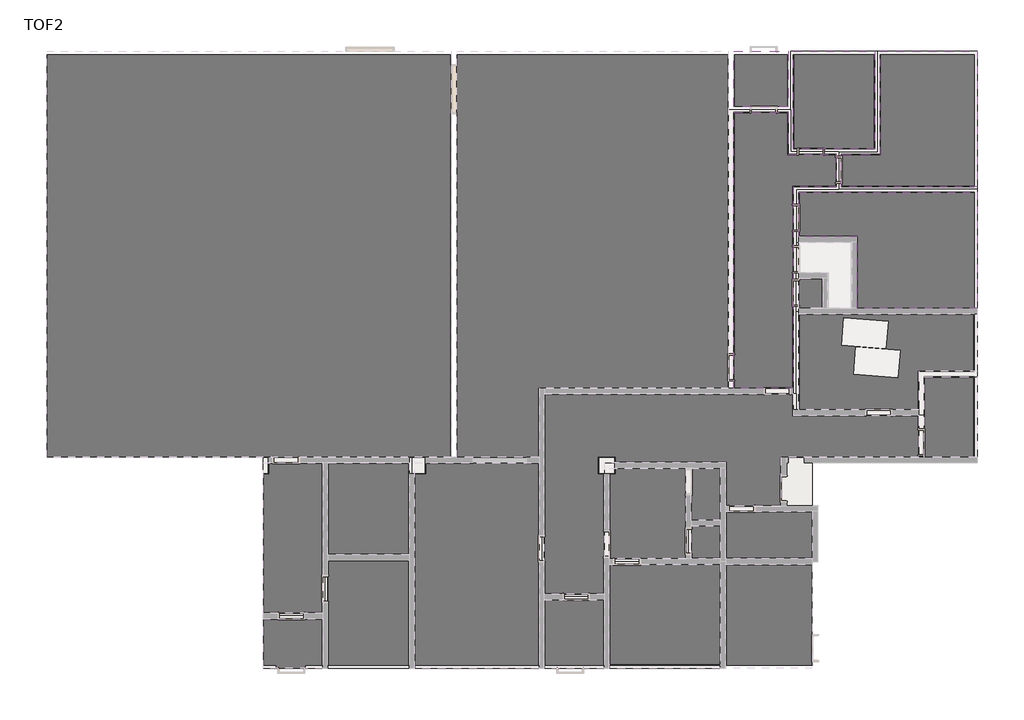
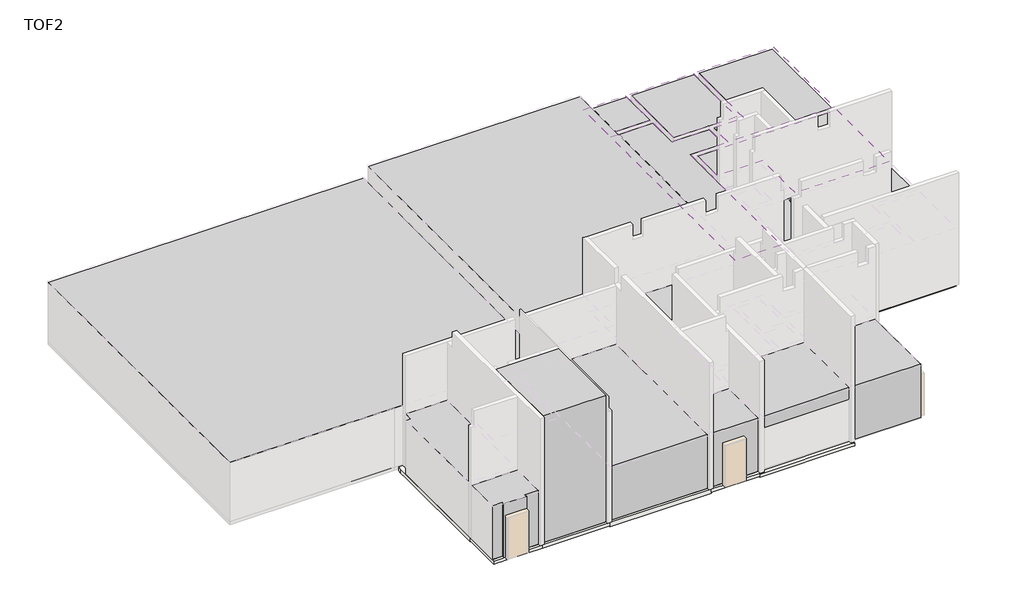
# One storey, part 5 of 5: 24 slabs, 23 proxies, 5 coverings.
"""IFC4 building model written with IfcOpenShell, lengths in millimetres."""

from ifc_helpers import new_model, si_unit, frame, origin, place, context, project, spatial, polyline, outline, extrude, faceted_brep, element, save

model = new_model("IFC4")

# Units and contexts
model_context = context("Model", 3, world=origin())
ifc_project = project(units=[si_unit("LENGTHUNIT", "METRE", prefix="MILLI")], contexts=[model_context])

# Site, building, storey
site = spatial("IfcSite", under=ifc_project)
building = spatial("IfcBuilding", under=site)
storey = spatial("IfcBuildingStorey", under=building, Name="TOF2", Elevation=1149.9618634)

# Proxies
placement = place(None, origin())
element("IfcBuildingElementProxy", 1, Name="Generic Models", at=placement, inside=storey, context=model_context, shape_type="SweptSolid", body=[
    extrude(outline(polyline([(18312.0, 23473.5208589), (33238.0, 23473.5208589), (33238.0, 8611.5208589), (26100.0, 8611.5208589), (18312.0, 8611.5208589), (18312.0, 23473.5208589)])), frame((0.0, 0.0, 1149.9618634), z_axis=(0.0, 0.0, 1.0), x_axis=(1.0, 0.0, 0.0)), (0.0, 0.0, 1.0), 3000.0),
])
element("IfcBuildingElementProxy", 2, Name="Generic Models", at=placement, inside=storey, context=model_context, shape_type="SweptSolid", body=[
    extrude(outline(polyline([(36488.0, 925.5208589), (31912.0, 925.5208589), (31912.0, 4899.0208589), (31912.0, 7987.5208589), (32312.0, 7987.5208589), (32312.0, 8387.5208589), (33350.0, 8387.5208589), (36488.0, 8387.5208589), (36488.0, 3443.8249516), (36488.0, 925.5208589)])), frame((0.0, 0.0, 1156.9618634), z_axis=(0.0, 0.0, 1.0), x_axis=(1.0, 0.0, 0.0)), (0.0, 0.0, 1.0), 2693.0),
])
element("IfcBuildingElementProxy", 3, Name="Generic Models", at=placement, inside=storey, context=model_context, shape_type="SweptSolid", body=[
    extrude(outline(polyline([(33462.0, 23473.5208589), (43488.0, 23473.5208589), (43488.0, 11161.5208589), (36488.0, 11161.5208589), (36488.0, 8611.5208589), (33462.0, 8611.5208589), (33462.0, 23473.5208589)])), frame((0.0, 0.0, 1149.9618634), z_axis=(0.0, 0.0, 1.0), x_axis=(1.0, 0.0, 0.0)), (0.0, 0.0, 1.0), 3500.0),
])
element("IfcBuildingElementProxy", 4, Name="Generic Models", at=placement, inside=storey, context=model_context, shape_type="SweptSolid", body=[
    extrude(outline(polyline([(39107.0, 932.5208589), (39107.0, 3443.8249516), (39107.0, 4642.5208589), (43193.0, 4642.5208589), (43193.0, 932.5208589), (39107.0, 932.5208589)])), frame((0.0, 0.0, 1199.9618634), z_axis=(0.0, 0.0, 1.0), x_axis=(1.0, 0.0, 0.0)), (0.0, 0.0, 1.0), 2650.0),
])
element("IfcBuildingElementProxy", 5, Name="Generic Models", at=placement, inside=storey, context=model_context, shape_type="SweptSolid", body=[
    extrude(outline(polyline([(39307.0, 7992.5208589), (39307.0, 8197.5208589), (41918.0, 8197.5208589), (41918.0, 6174.5208589), (41918.0, 4856.5208589), (39107.0, 4856.5208589), (39107.0, 7992.5208589), (39307.0, 7992.5208589)])), frame((0.0, 0.0, 1149.9618634), z_axis=(0.0, 0.0, 1.0), x_axis=(1.0, 0.0, 0.0)), (0.0, 0.0, 1.0), 2700.0),
])
element("IfcBuildingElementProxy", 6, Name="Generic Models", at=placement, inside=storey, context=model_context, shape_type="SweptSolid", body=[
    extrude(outline(polyline([(42132.0, 8197.5208589), (43193.0, 8197.5208589), (43193.0, 6699.5208589), (43193.0, 6281.5208589), (42132.0, 6281.5208589), (42132.0, 8197.5208589)])), frame((0.0, 0.0, 1199.9618634), z_axis=(0.0, 0.0, 1.0), x_axis=(1.0, 0.0, 0.0)), (0.0, 0.0, 1.0), 2650.0),
])
element("IfcBuildingElementProxy", 7, Name="Generic Models", at=placement, inside=storey, context=model_context, shape_type="SweptSolid", body=[
    extrude(outline(polyline([(43188.0, 4861.5208589), (42137.0, 4861.5208589), (42137.0, 6062.5208589), (43188.0, 6062.5208589), (43188.0, 4861.5208589)])), frame((0.0, 0.0, 1149.9618634), z_axis=(0.0, 0.0, 1.0), x_axis=(1.0, 0.0, 0.0)), (0.0, 0.0, 1.0), 2700.0),
])
element("IfcBuildingElementProxy", 8, Name="Generic Models", at=placement, inside=storey, context=model_context, shape_type="SweptSolid", body=[
    extrude(outline(polyline([(52567.0, 8606.5208589), (50732.0, 8606.5208589), (50732.0, 10249.5208589), (50732.0, 11567.5208589), (52567.0, 11567.5208589), (52567.0, 8606.5208589)])), frame((0.0, 0.0, 1199.9618634), z_axis=(0.0, 0.0, 1.0), x_axis=(1.0, 0.0, 0.0)), (0.0, 0.0, 1.0), 2650.0),
])
element("IfcBuildingElementProxy", 9, Name="Generic Models", at=placement, inside=storey, context=model_context, shape_type="SweptSolid", body=[
    extrude(outline(polyline([(52574.0, 23473.5208589), (52574.0, 18611.5208589), (47687.0, 18611.5208589), (47687.0, 19787.5208589), (49112.0, 19787.5208589), (49112.0, 23473.5208589), (52574.0, 23473.5208589)])), frame((0.0, 0.0, 1156.9618634), z_axis=(0.0, 0.0, 1.0), x_axis=(1.0, 0.0, 0.0)), (0.0, 0.0, 1.0), 2693.0),
])
element("IfcBuildingElementProxy", 10, Name="Generic Models", at=placement, inside=storey, context=model_context, shape_type="SweptSolid", body=[
    extrude(outline(polyline([(43712.0, 23473.5208589), (45688.0, 23473.5208589), (45688.0, 21561.5208589), (43712.0, 21561.5208589), (43712.0, 23473.5208589)])), frame((0.0, 0.0, 1156.9618634), z_axis=(0.0, 0.0, 1.0), x_axis=(1.0, 0.0, 0.0)), (0.0, 0.0, 1.0), 2693.0),
])
element("IfcBuildingElementProxy", 11, Name="Generic Models", at=placement, inside=storey, context=model_context, shape_type="SweptSolid", body=[
    extrude(outline(polyline([(45883.0, 11161.5208589), (43712.0, 11161.5208589), (43712.0, 21337.5208589), (45688.0, 21337.5208589), (45688.0, 19787.5208589), (47463.0, 19787.5208589), (47463.0, 18611.5208589), (45883.0, 18611.5208589), (45883.0, 16649.5208589), (45883.0, 15314.5208589), (45883.0, 13999.5208589), (45883.0, 11161.5208589)])), frame((0.0, 0.0, 1156.9618634), z_axis=(0.0, 0.0, 1.0), x_axis=(1.0, 0.0, 0.0)), (0.0, 0.0, 1.0), 2693.0),
])
element("IfcBuildingElementProxy", 12, Name="Generic Models", at=placement, inside=storey, context=model_context, shape_type="SweptSolid", body=[
    extrude(outline(polyline([(45912.0, 23473.5208589), (48888.0, 23473.5208589), (48888.0, 20011.5208589), (47575.0, 20011.5208589), (45912.0, 20011.5208589), (45912.0, 21449.5208589), (45912.0, 23473.5208589)])), frame((0.0, 0.0, 1156.9618634), z_axis=(0.0, 0.0, 1.0), x_axis=(1.0, 0.0, 0.0)), (0.0, 0.0, 1.0), 2693.0),
])
element("IfcBuildingElementProxy", 13, Name="Generic Models", at=placement, inside=storey, context=model_context, shape_type="SweptSolid", body=[
    extrude(outline(polyline([(50513.0, 10361.5208589), (46107.0, 10361.5208589), (46107.0, 13887.5208589), (52562.0, 13887.5208589), (52562.0, 11786.5208589), (50513.0, 11786.5208589), (50513.0, 10361.5208589)]), holes=[polyline([(47685.4846295, 12746.0331648), (49320.3101517, 12615.8582361), (49401.2726074, 13632.6399633), (47766.4470852, 13762.814892), (47685.4846295, 12746.0331648)]), polyline([(48126.4248192, 11673.6441948), (49761.2503413, 11543.4692661), (49842.212797, 12560.2509933), (48207.3872748, 12690.425922), (48126.4248192, 11673.6441948)])]), frame((0.0, 0.0, 1206.9618634), z_axis=(0.0, 0.0, 1.0), x_axis=(1.0, 0.0, 0.0)), (0.0, 0.0, 1.0), 2643.0),
])
element("IfcBuildingElementProxy", 14, Name="Generic Models", at=placement, inside=storey, context=model_context, shape_type="SweptSolid", body=[
    extrude(outline(polyline([(52574.0, 18387.5208589), (52574.0, 14111.5208589), (48262.0, 14111.5208589), (48262.0, 16761.5208589), (46107.0, 16761.5208589), (46107.0, 18387.5208589), (52574.0, 18387.5208589)])), frame((0.0, 0.0, 1156.9618634), z_axis=(0.0, 0.0, 1.0), x_axis=(1.0, 0.0, 0.0)), (0.0, 0.0, 1.0), 2693.0),
])
element("IfcBuildingElementProxy", 15, Name="Generic Models", at=placement, inside=storey, context=model_context, shape_type="SweptSolid", body=[
    extrude(outline(polyline([(46107.0, 14111.5208589), (46107.0, 15202.5208589), (46963.0, 15202.5208589), (46963.0, 14111.5208589), (46107.0, 14111.5208589)])), frame((0.0, 0.0, 1156.9618634), z_axis=(0.0, 0.0, 1.0), x_axis=(1.0, 0.0, 0.0)), (0.0, 0.0, 1.0), 2693.0),
])
element("IfcBuildingElementProxy", 16, Name="Generic Models", at=placement, inside=storey, context=model_context, shape_type="SweptSolid", body=[
    extrude(outline(polyline([(43412.0, 6587.5208589), (46588.0, 6587.5208589), (46588.0, 4861.5208589), (43412.0, 4861.5208589), (43412.0, 6587.5208589)])), frame((0.0, 0.0, 1156.9618634), z_axis=(0.0, 0.0, 1.0), x_axis=(1.0, 0.0, 0.0)), (0.0, 0.0, 1.0), 2693.0),
])
element("IfcBuildingElementProxy", 17, Name="Generic Models", at=placement, inside=storey, context=model_context, shape_type="SweptSolid", body=[
    extrude(outline(polyline([(46588.0, 925.5208589), (43412.0, 925.5208589), (43412.0, 4637.5208589), (46588.0, 4637.5208589), (46588.0, 925.5208589)])), frame((0.0, 0.0, 1156.9618634), z_axis=(0.0, 0.0, 1.0), x_axis=(1.0, 0.0, 0.0)), (0.0, 0.0, 1.0), 2693.0),
])
element("IfcBuildingElementProxy", 18, Name="Generic Models", at=placement, inside=storey, context=model_context, shape_type="SweptSolid", body=[
    extrude(outline(polyline([(31688.0, 925.5208589), (28712.0, 925.5208589), (28712.0, 4787.0208589), (31688.0, 4787.0208589), (31688.0, 925.5208589)])), frame((0.0, 0.0, 1156.9618634), z_axis=(0.0, 0.0, 1.0), x_axis=(1.0, 0.0, 0.0)), (0.0, 0.0, 1.0), 6343.0),
])
element("IfcBuildingElementProxy", 19, Name="Generic Models", at=placement, inside=storey, context=model_context, shape_type="SweptSolid", body=[
    extrude(outline(polyline([(28712.0, 8387.5208589), (31688.0, 8387.5208589), (31688.0, 7999.5208589), (31688.0, 5011.0208589), (28712.0, 5011.0208589), (28712.0, 8387.5208589)])), frame((0.0, 0.0, 1156.9618634), z_axis=(0.0, 0.0, 1.0), x_axis=(1.0, 0.0, 0.0)), (0.0, 0.0, 1.0), 2693.0),
])
element("IfcBuildingElementProxy", 20, Name="Generic Models", at=placement, inside=storey, context=model_context, shape_type="Brep", body=[
    faceted_brep([(26787.0, 925.5208589, 1156.9618634), (26850.0, 925.5208589, 1156.9618634), (26850.0, 925.5208589, 1149.9618634), (26787.0, 925.5208589, 1149.9618634), (26850.0, 799.5208589, 1156.9618634), (26312.0, 925.5208589, 1156.9618634), (26312.0, 2625.0208589, 1156.9618634), (28488.0, 2625.0208589, 1156.9618634), (28488.0, 925.5208589, 1156.9618634), (27855.0, 925.5208589, 1156.9618634), (27855.0, 799.5208589, 1156.9618634), (26787.0, 925.5208589, 3849.9618634), (26312.0, 925.5208589, 3849.9618634), (26850.0, 799.5208589, 1149.9618634), (26787.0, 799.5208589, 1149.9618634), (26787.0, 799.5208589, 3849.9618634), (27855.0, 799.5208589, 3849.9618634), (26312.0, 2625.0208589, 3849.9618634), (28488.0, 2625.0208589, 3849.9618634), (28488.0, 925.5208589, 3849.9618634), (27855.0, 925.5208589, 3849.9618634)], [[[0, 1, 2, 3]], [[4, 1, 0, 5, 6, 7, 8, 9, 10]], [[11, 12, 5, 0]], [[1, 4, 13, 2]], [[14, 3, 2, 13]], [[3, 14, 15, 11, 0]], [[15, 14, 13, 4, 10, 16]], [[12, 17, 6, 5]], [[17, 18, 7, 6]], [[18, 19, 8, 7]], [[19, 20, 9, 8]], [[20, 16, 10, 9]], [[11, 15, 16, 20, 19, 18, 17, 12]]]),
])
element("IfcBuildingElementProxy", 21, Name="Generic Models", at=placement, inside=storey, context=model_context, shape_type="SweptSolid", body=[
    extrude(outline(polyline([(26512.0, 7987.5208589), (26512.0, 8387.5208589), (28488.0, 8387.5208589), (28488.0, 4899.0208589), (28488.0, 2849.0208589), (26312.0, 2849.0208589), (26312.0, 7987.5208589), (26512.0, 7987.5208589)])), frame((0.0, 0.0, 1156.9618634), z_axis=(0.0, 0.0, 1.0), x_axis=(1.0, 0.0, 0.0)), (0.0, 0.0, 1.0), 2693.0),
])
element("IfcBuildingElementProxy", 22, Name="Generic Models", at=placement, inside=storey, context=model_context, shape_type="SweptSolid", body=[
    extrude(outline(polyline([(39312.0, 8416.5208589), (39312.0, 8611.5208589), (38688.0, 8611.5208589), (38688.0, 7987.5208589), (38888.0, 7987.5208589), (38888.0, 3555.8249516), (36712.0, 3555.8249516), (36712.0, 8499.5208589), (36712.0, 10937.5208589), (43600.0, 10937.5208589), (45883.0, 10937.5208589), (45883.0, 10137.5208589), (50513.0, 10137.5208589), (50513.0, 8611.5208589), (45428.0, 8611.5208589), (45428.0, 6811.5208589), (43412.0, 6811.5208589), (43412.0, 8416.5208589), (39312.0, 8416.5208589)])), frame((0.0, 0.0, 1156.9618634), z_axis=(0.0, 0.0, 1.0), x_axis=(1.0, 0.0, 0.0)), (0.0, 0.0, 1.0), 2693.0),
])
element("IfcBuildingElementProxy", 23, Name="Generic Models", at=placement, inside=storey, context=model_context, shape_type="SweptSolid", body=[
    extrude(outline(polyline([(38888.0, 925.5208589), (36712.0, 925.5208589), (36712.0, 3331.8249516), (38888.0, 3331.8249516), (38888.0, 925.5208589)])), frame((0.0, 0.0, 1156.9618634), z_axis=(0.0, 0.0, 1.0), x_axis=(1.0, 0.0, 0.0)), (0.0, 0.0, 1.0), 2693.0),
])

# Coverings
element("IfcCovering", 24, ObjectType="H_CE_AR_B09_Acoustic Ceiling_T Bar_600x600x9T", at=placement, inside=storey, context=model_context, shape_type="SweptSolid", body=[
    extrude(outline(polyline([(43700.0, 23599.5208589), (45700.0, 23599.5208589), (45700.0, 21549.5208589), (43700.0, 21549.5208589), (43700.0, 23599.5208589)])), frame((0.0, 0.0, 3849.9618634), z_axis=(0.0, 0.0, 1.0), x_axis=(1.0, 0.0, 0.0)), (0.0, 0.0, 1.0), 9.0),
])
element("IfcCovering", 25, ObjectType="H_CE_AR_B09_Acoustic Ceiling_T Bar_600x600x9T", at=placement, inside=storey, context=model_context, shape_type="SweptSolid", body=[
    extrude(outline(polyline([(45900.0, 23599.5208589), (48900.0, 23599.5208589), (48900.0, 19999.5208589), (45900.0, 19999.5208589), (45900.0, 23599.5208589)])), frame((0.0, 0.0, 3849.9618634), z_axis=(0.0, 0.0, 1.0), x_axis=(1.0, 0.0, 0.0)), (0.0, 0.0, 1.0), 9.0),
])
element("IfcCovering", 26, ObjectType="H_CE_AR_B09_Acoustic Ceiling_T Bar_600x600x9T", at=placement, inside=storey, context=model_context, shape_type="SweptSolid", body=[
    extrude(outline(polyline([(49100.0, 23599.5208589), (52700.0, 23599.5208589), (52700.0, 18599.5208589), (47675.0, 18599.5208589), (47675.0, 19799.5208589), (49100.0, 19799.5208589), (49100.0, 23599.5208589)])), frame((0.0, 0.0, 3849.9618634), z_axis=(0.0, 0.0, 1.0), x_axis=(1.0, 0.0, 0.0)), (0.0, 0.0, 1.0), 9.0),
])
element("IfcCovering", 27, ObjectType="H_CE_AR_B09_Acoustic Ceiling_T Bar_600x600x9T", at=placement, inside=storey, context=model_context, shape_type="SweptSolid", body=[
    extrude(outline(polyline([(45895.0, 18599.5208589), (45895.0, 11149.5208589), (43700.0, 11149.5208589), (43700.0, 21349.5208589), (45700.0, 21349.5208589), (45700.0, 19799.5208589), (47475.0, 19799.5208589), (47475.0, 18599.5208589), (45895.0, 18599.5208589)])), frame((0.0, 0.0, 3849.9618634), z_axis=(0.0, 0.0, 1.0), x_axis=(1.0, 0.0, 0.0)), (0.0, 0.0, 1.0), 9.0),
])
element("IfcCovering", 28, ObjectType="H_CE_AR_B09_Acoustic Ceiling_T Bar_600x600x9T", at=placement, inside=storey, context=model_context, shape_type="SweptSolid", body=[
    extrude(outline(polyline([(52700.0, 18399.5208589), (52700.0, 14099.5208589), (48250.0, 14099.5208589), (48250.0, 16749.5208589), (46095.0, 16749.5208589), (46095.0, 18399.5208589), (52700.0, 18399.5208589)])), frame((0.0, 0.0, 3849.9618634), z_axis=(0.0, 0.0, 1.0), x_axis=(1.0, 0.0, 0.0)), (0.0, 0.0, 1.0), 9.0),
])

# Slabs
element("IfcSlab", 29, ObjectType="H_SF_AR_S17_SOG T200_GS1", at=placement, inside=storey, context=model_context, shape_type="Brep", body=[
    faceted_brep([(33350.0, 8599.5208589, 949.9618634), (36600.0, 8599.5208589, 949.9618634), (36600.0, 3443.8249516, 949.9618634), (36600.0, 925.5208589, 949.9618634), (36600.0, 799.5208589, 949.9618634), (31800.0, 799.5208589, 949.9618634), (31800.0, 925.5208589, 949.9618634), (31800.0, 4899.0208589, 949.9618634), (31800.0, 8599.5208589, 949.9618634), (32300.0, 8599.5208589, 949.9618634), (33350.0, 8599.5208589, 1149.9618634), (31800.0, 8599.5208589, 1149.9618634), (31800.0, 4899.0208589, 1149.9618634), (31800.0, 799.5208589, 1149.9618634), (31900.0, 799.5208589, 1149.9618634), (36500.0, 799.5208589, 1149.9618634), (36600.0, 799.5208589, 1149.9618634), (36600.0, 3443.8249516, 1149.9618634), (36600.0, 8599.5208589, 1149.9618634), (36500.0, 8599.5208589, 1149.9618634), (36600.0, 799.5208589, 999.9618634), (31800.0, 799.5208589, 999.9618634)], [[[0, 1, 2, 3, 4, 5, 6, 7, 8, 9]], [[10, 11, 12, 13, 14, 15, 16, 17, 18, 19]], [[1, 0, 10, 19, 18]], [[2, 1, 18, 17]], [[4, 3, 2, 17, 16, 20]], [[5, 4, 20, 16, 15, 14, 13, 21]], [[7, 6, 5, 21, 13, 12]], [[8, 7, 12, 11]], [[0, 9, 8, 11, 10]]]),
])
element("IfcSlab", 30, ObjectType="H_SF_AR_S17_SOG T150_GS1", at=placement, inside=storey, context=model_context, shape_type="Brep", body=[
    faceted_brep([(38900.0, 799.5208589, 949.9618634), (38900.0, 925.5208589, 949.9618634), (38900.0, 3443.8249516, 949.9618634), (38900.0, 4749.5208589, 949.9618634), (42025.0, 4749.5208589, 949.9618634), (43400.0, 4749.5208589, 949.9618634), (43400.0, 4649.5208589, 949.9618634), (43400.0, 925.5208589, 949.9618634), (43400.0, 799.5208589, 949.9618634), (43200.0, 799.5208589, 949.9618634), (38900.0, 799.5208589, 1099.9618634), (43200.0, 799.5208589, 1099.9618634), (43400.0, 799.5208589, 1099.9618634), (43400.0, 925.5208589, 1099.9618634), (43400.0, 4749.5208589, 1099.9618634), (42025.0, 4749.5208589, 1099.9618634), (38900.0, 4749.5208589, 1099.9618634), (38900.0, 3443.8249516, 1099.9618634), (38900.0, 925.5208589, 1099.9618634), (38900.0, 799.5208589, 999.9618634)], [[[0, 1, 2, 3, 4, 5, 6, 7, 8, 9]], [[10, 11, 12, 13, 14, 15, 16, 17, 18]], [[2, 1, 0, 19, 10, 18, 17]], [[3, 2, 17, 16]], [[4, 3, 16, 15]], [[5, 4, 15, 14]], [[8, 7, 6, 5, 14, 13, 12]], [[0, 9, 8, 12, 11, 10, 19]]]),
])
element("IfcSlab", 31, ObjectType="H_SF_AR_S17_SOG T150_GS1", at=placement, inside=storey, context=model_context, shape_type="SweptSolid", body=[
    extrude(outline(polyline([(38900.0, 4749.5208589), (38900.0, 8404.5208589), (42025.0, 8404.5208589), (42025.0, 6174.5208589), (42025.0, 4749.5208589), (38900.0, 4749.5208589)])), frame((0.0, 0.0, 949.9618634), z_axis=(0.0, 0.0, 1.0), x_axis=(1.0, 0.0, 0.0)), (0.0, 0.0, 1.0), 150.0),
])
element("IfcSlab", 32, ObjectType="H_SF_AR_S17_SOG T200_GS1", at=placement, inside=storey, context=model_context, shape_type="Brep", body=[
    faceted_brep([(42025.0, 8404.5208589, 949.9618634), (43400.0, 8404.5208589, 949.9618634), (43400.0, 6699.5208589, 949.9618634), (43400.0, 6174.5208589, 949.9618634), (42025.0, 6174.5208589, 949.9618634), (42025.0, 8404.5208589, 1149.9618634), (42025.0, 6174.5208589, 1149.9618634), (43400.0, 6174.5208589, 1149.9618634), (43400.0, 6699.5208589, 1149.9618634), (43400.0, 8404.5208589, 1149.9618634), (42025.0, 8404.5208589, 1099.9618634), (43400.0, 6174.5208589, 1099.9618634), (42025.0, 6174.5208589, 1099.9618634)], [[[0, 1, 2, 3, 4]], [[5, 6, 7, 8, 9]], [[1, 0, 10, 5, 9]], [[2, 1, 9, 8]], [[3, 2, 8, 7, 11]], [[4, 3, 11, 7, 6, 12]], [[0, 4, 12, 6, 5, 10]]]),
])
element("IfcSlab", 33, ObjectType="H_SF_AR_S17_SOG T150_GS1", at=placement, inside=storey, context=model_context, shape_type="Brep", body=[
    faceted_brep([(43400.0, 4749.5208589, 949.9618634), (42025.0, 4749.5208589, 949.9618634), (42025.0, 6174.5208589, 949.9618634), (43400.0, 6174.5208589, 949.9618634), (43400.0, 4849.5208589, 949.9618634), (43400.0, 4749.5208589, 1099.9618634), (43400.0, 4849.5208589, 1099.9618634), (43400.0, 6174.5208589, 1099.9618634), (42025.0, 6174.5208589, 1099.9618634), (42025.0, 4749.5208589, 1099.9618634)], [[[0, 1, 2, 3, 4]], [[5, 6, 7, 8, 9]], [[1, 0, 5, 9]], [[2, 1, 9, 8]], [[3, 2, 8, 7]], [[0, 4, 3, 7, 6, 5]]]),
])
element("IfcSlab", 34, ObjectType="H_SF_AR_S17_SOG T150_GS1", at=placement, inside=storey, context=model_context, shape_type="Brep", body=[
    faceted_brep([(52700.0, 8599.5208589, 949.9618634), (52574.0, 8599.5208589, 949.9618634), (50725.0, 8599.5208589, 949.9618634), (50725.0, 10149.5208589, 949.9618634), (50725.0, 10249.5208589, 949.9618634), (50725.0, 11574.5208589, 949.9618634), (52574.0, 11574.5208589, 949.9618634), (52700.0, 11574.5208589, 949.9618634), (52700.0, 8599.5208589, 1099.9618634), (52700.0, 11574.5208589, 1099.9618634), (52574.0, 11574.5208589, 1099.9618634), (50725.0, 11574.5208589, 1099.9618634), (50725.0, 10249.5208589, 1099.9618634), (50725.0, 8599.5208589, 1099.9618634), (52574.0, 8599.5208589, 1099.9618634), (50725.0, 11574.5208589, 999.9618634), (52700.0, 11574.5208589, 999.9618634)], [[[0, 1, 2, 3, 4, 5, 6, 7]], [[8, 9, 10, 11, 12, 13, 14]], [[2, 1, 0, 8, 14, 13]], [[4, 3, 2, 13, 12]], [[5, 4, 12, 11, 15]], [[7, 6, 5, 15, 11, 10, 9, 16]], [[0, 7, 16, 9, 8]]]),
])
element("IfcSlab", 35, ObjectType="H_SF_AR_S17_SOG T150_GS1", at=placement, inside=storey, context=model_context, shape_type="Brep", body=[
    faceted_brep([(52700.0, 18499.5208589, 999.9618634), (47575.0, 18499.5208589, 999.9618634), (47575.0, 19899.5208589, 999.9618634), (49000.0, 19899.5208589, 999.9618634), (49000.0, 23599.5208589, 999.9618634), (49100.0, 23599.5208589, 999.9618634), (52574.0, 23599.5208589, 999.9618634), (52700.0, 23599.5208589, 999.9618634), (52700.0, 18599.5208589, 999.9618634), (52700.0, 18499.5208589, 1149.9618634), (52700.0, 18599.5208589, 1149.9618634), (52700.0, 23599.5208589, 1149.9618634), (52574.0, 23599.5208589, 1149.9618634), (49100.0, 23599.5208589, 1149.9618634), (49000.0, 23599.5208589, 1149.9618634), (49000.0, 19899.5208589, 1149.9618634), (47575.0, 19899.5208589, 1149.9618634), (47575.0, 18499.5208589, 1149.9618634)], [[[0, 1, 2, 3, 4, 5, 6, 7, 8]], [[9, 10, 11, 12, 13, 14, 15, 16, 17]], [[1, 0, 9, 17]], [[2, 1, 17, 16]], [[3, 2, 16, 15]], [[4, 3, 15, 14]], [[7, 6, 5, 4, 14, 13, 12, 11]], [[0, 8, 7, 11, 10, 9]]]),
])
element("IfcSlab", 36, ObjectType="H_SF_AR_S17_SOG T150_GS1", at=placement, inside=storey, context=model_context, shape_type="Brep", body=[
    faceted_brep([(46000.0, 10949.5208589, 999.9618634), (43500.0, 10949.5208589, 999.9618634), (43500.0, 11149.5208589, 999.9618634), (43500.0, 21449.5208589, 999.9618634), (43700.0, 21449.5208589, 999.9618634), (45800.0, 21449.5208589, 999.9618634), (45800.0, 19899.5208589, 999.9618634), (47575.0, 19899.5208589, 999.9618634), (47575.0, 18499.5208589, 999.9618634), (46000.0, 18499.5208589, 999.9618634), (46000.0, 16649.5208589, 999.9618634), (46000.0, 16549.5208589, 999.9618634), (46000.0, 15414.5208589, 999.9618634), (46000.0, 15412.0208589, 999.9618634), (46000.0, 15314.5208589, 999.9618634), (46000.0, 13999.5208589, 999.9618634), (46000.0, 11149.5208589, 999.9618634), (46000.0, 10949.5208589, 1149.9618634), (46000.0, 13999.5208589, 1149.9618634), (46000.0, 15314.5208589, 1149.9618634), (46000.0, 15412.0208589, 1149.9618634), (46000.0, 16412.0208589, 1149.9618634), (46000.0, 16549.5208589, 1149.9618634), (46000.0, 16649.5208589, 1149.9618634), (46000.0, 18499.5208589, 1149.9618634), (47575.0, 18499.5208589, 1149.9618634), (47575.0, 19899.5208589, 1149.9618634), (45800.0, 19899.5208589, 1149.9618634), (45800.0, 21449.5208589, 1149.9618634), (43700.0, 21449.5208589, 1149.9618634), (43500.0, 21449.5208589, 1149.9618634), (43500.0, 12424.5208589, 1149.9618634), (43500.0, 11424.5208589, 1149.9618634), (43500.0, 11149.5208589, 1149.9618634), (43500.0, 10949.5208589, 1149.9618634), (44800.0, 10949.5208589, 1149.9618634), (45800.0, 10949.5208589, 1149.9618634), (45895.0, 10949.5208589, 1149.9618634)], [[[0, 1, 2, 3, 4, 5, 6, 7, 8, 9, 10, 11, 12, 13, 14, 15, 16]], [[17, 18, 19, 20, 21, 22, 23, 24, 25, 26, 27, 28, 29, 30, 31, 32, 33, 34, 35, 36, 37]], [[1, 0, 17, 37, 36, 35, 34]], [[3, 2, 1, 34, 33, 32, 31, 30]], [[5, 4, 3, 30, 29, 28]], [[6, 5, 28, 27]], [[7, 6, 27, 26]], [[8, 7, 26, 25]], [[9, 8, 25, 24]], [[10, 9, 24, 23]], [[14, 13, 12, 11, 10, 23, 22, 21, 20, 19]], [[15, 14, 19, 18]], [[0, 16, 15, 18, 17]]]),
])
element("IfcSlab", 37, ObjectType="H_SF_AR_S17_SOG T150_GS1", at=placement, inside=storey, context=model_context, shape_type="Brep", body=[
    faceted_brep([(47575.0, 19899.5208589, 999.9618634), (45800.0, 19899.5208589, 999.9618634), (45800.0, 21449.5208589, 999.9618634), (45800.0, 23599.5208589, 999.9618634), (45900.0, 23599.5208589, 999.9618634), (48900.0, 23599.5208589, 999.9618634), (49000.0, 23599.5208589, 999.9618634), (49000.0, 19899.5208589, 999.9618634), (45800.0, 19899.5208589, 1149.9618634), (47575.0, 19899.5208589, 1149.9618634), (49000.0, 19899.5208589, 1149.9618634), (49000.0, 23599.5208589, 1149.9618634), (48900.0, 23599.5208589, 1149.9618634), (45900.0, 23599.5208589, 1149.9618634), (45800.0, 23599.5208589, 1149.9618634), (45800.0, 21449.5208589, 1149.9618634)], [[[0, 1, 2, 3, 4, 5, 6, 7]], [[8, 9, 10, 11, 12, 13, 14, 15]], [[1, 0, 9, 8]], [[2, 1, 8, 15]], [[3, 2, 15, 14]], [[6, 5, 4, 3, 14, 13, 12, 11]], [[7, 6, 11, 10]], [[0, 7, 10, 9]]]),
])
element("IfcSlab", 38, ObjectType="H_SF_AR_S17_SOG T150_GS1", at=placement, inside=storey, context=model_context, shape_type="Brep", body=[
    faceted_brep([(50725.0, 10149.5208589, 999.9618634), (50525.0, 10149.5208589, 999.9618634), (46000.0, 10149.5208589, 999.9618634), (46000.0, 10349.5208589, 999.9618634), (46000.0, 10949.5208589, 999.9618634), (46000.0, 11049.5208589, 999.9618634), (46000.0, 11149.5208589, 999.9618634), (46000.0, 13999.5208589, 999.9618634), (47075.0, 13999.5208589, 999.9618634), (47175.0, 13999.5208589, 999.9618634), (48050.0, 13999.5208589, 999.9618634), (48150.0, 13999.5208589, 999.9618634), (52700.0, 13999.5208589, 999.9618634), (52700.0, 11774.5208589, 999.9618634), (52700.0, 11574.5208589, 999.9618634), (50725.0, 11574.5208589, 999.9618634), (50725.0, 10249.5208589, 999.9618634), (46000.0, 10149.5208589, 1149.9618634), (50725.0, 10149.5208589, 1149.9618634), (50725.0, 11574.5208589, 1149.9618634), (52700.0, 11574.5208589, 1149.9618634), (52700.0, 11774.5208589, 1149.9618634), (52700.0, 13899.5208589, 1149.9618634), (52700.0, 13999.5208589, 1149.9618634), (48150.0, 13999.5208589, 1149.9618634), (48050.0, 13999.5208589, 1149.9618634), (47175.0, 13999.5208589, 1149.9618634), (47075.0, 13999.5208589, 1149.9618634), (46000.0, 13999.5208589, 1149.9618634), (46000.0, 11049.5208589, 1149.9618634), (46000.0, 10949.5208589, 1149.9618634), (50725.0, 10149.5208589, 1099.9618634), (52700.0, 11574.5208589, 1099.9618634), (50725.0, 11574.5208589, 1099.9618634)], [[[0, 1, 2, 3, 4, 5, 6, 7, 8, 9, 10, 11, 12, 13, 14, 15, 16]], [[17, 18, 19, 20, 21, 22, 23, 24, 25, 26, 27, 28, 29, 30]], [[2, 1, 0, 31, 18, 17]], [[2, 17, 30, 29, 5, 4, 3]], [[7, 6, 5, 29, 28]], [[8, 7, 28, 27]], [[11, 10, 9, 8, 27, 26, 25, 24]], [[12, 11, 24, 23]], [[14, 13, 12, 23, 22, 21, 20, 32]], [[15, 14, 32, 20, 19, 33]], [[19, 18, 31, 0, 16, 15, 33]]]),
])
element("IfcSlab", 39, ObjectType="H_SF_AR_S17_SOG T150_GS1", at=placement, inside=storey, context=model_context, shape_type="Brep", body=[
    faceted_brep([(46000.0, 18499.5208589, 999.9618634), (47575.0, 18499.5208589, 999.9618634), (52700.0, 18499.5208589, 999.9618634), (52700.0, 18399.5208589, 999.9618634), (52700.0, 13999.5208589, 999.9618634), (48050.0, 13999.5208589, 999.9618634), (48050.0, 16549.5208589, 999.9618634), (46095.0, 16549.5208589, 999.9618634), (46000.0, 16549.5208589, 999.9618634), (46000.0, 16649.5208589, 999.9618634), (47575.0, 18499.5208589, 1149.9618634), (46000.0, 18499.5208589, 1149.9618634), (46000.0, 16649.5208589, 1149.9618634), (46000.0, 16549.5208589, 1149.9618634), (46095.0, 16549.5208589, 1149.9618634), (48050.0, 16549.5208589, 1149.9618634), (48050.0, 13999.5208589, 1149.9618634), (52700.0, 13999.5208589, 1149.9618634), (52700.0, 14099.5208589, 1149.9618634), (52700.0, 18399.5208589, 1149.9618634), (52700.0, 18499.5208589, 1149.9618634), (46000.0, 16549.5208589, 1099.9618634), (48050.0, 13999.5208589, 1099.9618634), (48050.0, 16549.5208589, 1099.9618634)], [[[0, 1, 2, 3, 4, 5, 6, 7, 8, 9]], [[10, 11, 12, 13, 14, 15, 16, 17, 18, 19, 20]], [[11, 0, 9, 8, 21, 13, 12]], [[1, 0, 11, 10]], [[2, 1, 10, 20]], [[4, 3, 2, 20, 19, 18, 17]], [[5, 4, 17, 16, 22]], [[6, 5, 22, 16, 15, 23]], [[8, 7, 6, 23, 15, 14, 13, 21]]]),
])
element("IfcSlab", 40, ObjectType="H_SF_AR_S17_SOG T150_GS1", at=placement, inside=storey, context=model_context, shape_type="Brep", body=[
    faceted_brep([(46000.0, 15414.5208589, 949.9618634), (46000.0, 16549.5208589, 949.9618634), (46095.0, 16549.5208589, 949.9618634), (48050.0, 16549.5208589, 949.9618634), (48050.0, 13999.5208589, 949.9618634), (47175.0, 13999.5208589, 949.9618634), (47175.0, 15414.5208589, 949.9618634), (46095.0, 15414.5208589, 949.9618634), (46000.0, 16549.5208589, 1099.9618634), (46000.0, 15414.5208589, 1099.9618634), (46095.0, 15414.5208589, 1099.9618634), (47175.0, 15414.5208589, 1099.9618634), (47175.0, 13999.5208589, 1099.9618634), (48050.0, 13999.5208589, 1099.9618634), (48050.0, 16549.5208589, 1099.9618634), (46095.0, 16549.5208589, 1099.9618634), (46000.0, 15414.5208589, 999.9618634), (46000.0, 16549.5208589, 999.9618634), (48050.0, 16549.5208589, 999.9618634), (48050.0, 13999.5208589, 999.9618634), (47175.0, 13999.5208589, 999.9618634)], [[[0, 1, 2, 3, 4, 5, 6, 7]], [[8, 9, 10, 11, 12, 13, 14, 15]], [[1, 0, 16, 9, 8, 17]], [[3, 2, 1, 17, 8, 15, 14, 18]], [[4, 3, 18, 14, 13, 19]], [[5, 4, 19, 13, 12, 20]], [[6, 5, 20, 12, 11]], [[0, 7, 6, 11, 10, 9, 16]]]),
])
element("IfcSlab", 41, ObjectType="H_SF_AR_S17_SOG T150_GS1", at=placement, inside=storey, context=model_context, shape_type="Brep", body=[
    faceted_brep([(46000.0, 15412.0208589, 999.9618634), (46095.0, 15412.0208589, 999.9618634), (47175.0, 15412.0208589, 999.9618634), (47175.0, 13999.5208589, 999.9618634), (46000.0, 13999.5208589, 999.9618634), (46000.0, 15314.5208589, 999.9618634), (47175.0, 15412.0208589, 1149.9618634), (46095.0, 15412.0208589, 1149.9618634), (46000.0, 15412.0208589, 1149.9618634), (46000.0, 15314.5208589, 1149.9618634), (46000.0, 13999.5208589, 1149.9618634), (47175.0, 13999.5208589, 1149.9618634), (47175.0, 15214.5208589, 1149.9618634), (47175.0, 15412.0208589, 1099.9618634), (47175.0, 13999.5208589, 1099.9618634)], [[[0, 1, 2, 3, 4, 5]], [[6, 7, 8, 9, 10, 11, 12]], [[8, 0, 5, 4, 10, 9]], [[2, 1, 0, 8, 7, 6, 13]], [[3, 2, 13, 6, 12, 11, 14]], [[4, 3, 14, 11, 10]]]),
])
element("IfcSlab", 42, ObjectType="H_SF_AR_S17_SOG T150_GS1", at=placement, inside=storey, context=model_context, shape_type="Brep", body=[
    faceted_brep([(31800.0, 4899.0208589, 999.9618634), (31800.0, 925.5208589, 999.9618634), (31800.0, 799.5208589, 999.9618634), (28600.0, 799.5208589, 999.9618634), (28600.0, 2737.0208589, 999.9618634), (28600.0, 4899.0208589, 999.9618634), (31800.0, 4899.0208589, 1149.9618634), (28600.0, 4899.0208589, 1149.9618634), (28600.0, 2737.0208589, 1149.9618634), (28600.0, 799.5208589, 1149.9618634), (28700.0, 799.5208589, 1149.9618634), (31700.0, 799.5208589, 1149.9618634), (31800.0, 799.5208589, 1149.9618634)], [[[0, 1, 2, 3, 4, 5]], [[6, 7, 8, 9, 10, 11, 12]], [[2, 1, 0, 6, 12]], [[3, 2, 12, 11, 10, 9]], [[4, 3, 9, 8]], [[5, 4, 8, 7]], [[0, 5, 7, 6]]]),
])
element("IfcSlab", 43, ObjectType="H_SF_AR_S17_SOG T200_GS1", at=placement, inside=storey, context=model_context, shape_type="Brep", body=[
    faceted_brep([(28600.0, 8599.5208589, 949.9618634), (31700.0, 8599.5208589, 949.9618634), (31800.0, 8599.5208589, 949.9618634), (31800.0, 4899.0208589, 949.9618634), (28600.0, 4899.0208589, 949.9618634), (28600.0, 8599.5208589, 1149.9618634), (28600.0, 4899.0208589, 1149.9618634), (31800.0, 4899.0208589, 1149.9618634), (31800.0, 8599.5208589, 1149.9618634), (31800.0, 4899.0208589, 999.9618634), (28600.0, 4899.0208589, 999.9618634)], [[[0, 1, 2, 3, 4]], [[5, 6, 7, 8]], [[2, 1, 0, 5, 8]], [[3, 2, 8, 7, 9]], [[4, 3, 9, 7, 6, 10]], [[0, 4, 10, 6, 5]]]),
])
element("IfcSlab", 44, ObjectType="H_SF_AR_S17_SOG T150_GS1", at=placement, inside=storey, context=model_context, shape_type="Brep", body=[
    faceted_brep([(26300.0, 799.5208589, 999.9618634), (26300.0, 925.5208589, 999.9618634), (26300.0, 2737.0208589, 999.9618634), (26500.0, 2737.0208589, 999.9618634), (28600.0, 2737.0208589, 999.9618634), (28600.0, 799.5208589, 999.9618634), (27855.0, 799.5208589, 999.9618634), (26850.0, 799.5208589, 999.9618634), (26724.0, 799.5208589, 999.9618634), (26500.0, 799.5208589, 999.9618634), (26300.0, 799.5208589, 1149.9618634), (26724.0, 799.5208589, 1149.9618634), (26850.0, 799.5208589, 1149.9618634), (27850.0, 799.5208589, 1149.9618634), (27855.0, 799.5208589, 1149.9618634), (28500.0, 799.5208589, 1149.9618634), (28600.0, 799.5208589, 1149.9618634), (28600.0, 2737.0208589, 1149.9618634), (26300.0, 2737.0208589, 1149.9618634), (26300.0, 925.5208589, 1149.9618634)], [[[0, 1, 2, 3, 4, 5, 6, 7, 8, 9]], [[10, 11, 12, 13, 14, 15, 16, 17, 18, 19]], [[2, 1, 0, 10, 19, 18]], [[4, 3, 2, 18, 17]], [[5, 4, 17, 16]], [[0, 9, 8, 7, 6, 5, 16, 15, 14, 13, 12, 11, 10]]]),
])
element("IfcSlab", 45, ObjectType="H_SF_AR_S17_SOG T200_GS1", at=placement, inside=storey, context=model_context, shape_type="Brep", body=[
    faceted_brep([(26300.0, 8599.5208589, 949.9618634), (26500.0, 8599.5208589, 949.9618634), (28600.0, 8599.5208589, 949.9618634), (28600.0, 4899.0208589, 949.9618634), (28600.0, 2737.0208589, 949.9618634), (26500.0, 2737.0208589, 949.9618634), (26300.0, 2737.0208589, 949.9618634), (26300.0, 7999.5208589, 949.9618634), (26300.0, 8397.9255867, 949.9618634), (26300.0, 8599.5208589, 1149.9618634), (26300.0, 8397.9255867, 1149.9618634), (26300.0, 2737.0208589, 1149.9618634), (28600.0, 2737.0208589, 1149.9618634), (28600.0, 4899.0208589, 1149.9618634), (28600.0, 8599.5208589, 1149.9618634), (27650.0, 8599.5208589, 1149.9618634), (26650.0, 8599.5208589, 1149.9618634), (28600.0, 2737.0208589, 999.9618634), (26300.0, 2737.0208589, 999.9618634)], [[[0, 1, 2, 3, 4, 5, 6, 7, 8]], [[9, 10, 11, 12, 13, 14, 15, 16]], [[2, 1, 0, 9, 16, 15, 14]], [[3, 2, 14, 13]], [[4, 3, 13, 12, 17]], [[6, 5, 4, 17, 12, 11, 18]], [[8, 7, 6, 18, 11, 10]], [[0, 8, 10, 9]]]),
])
element("IfcSlab", 46, ObjectType="H_SF_AR_S17_SOG T200_GS1", at=placement, inside=storey, context=model_context, shape_type="Brep", body=[
    faceted_brep([(36600.0, 8499.5208589, 949.9618634), (36600.0, 8599.5208589, 949.9618634), (36600.0, 10799.5208589, 949.9618634), (36600.0, 11149.5208589, 949.9618634), (43500.0, 11149.5208589, 949.9618634), (43600.0, 11149.5208589, 949.9618634), (43700.0, 11149.5208589, 949.9618634), (45895.0, 11149.5208589, 949.9618634), (46000.0, 11149.5208589, 949.9618634), (46000.0, 10349.5208589, 949.9618634), (46000.0, 10149.5208589, 949.9618634), (50525.0, 10149.5208589, 949.9618634), (50725.0, 10149.5208589, 949.9618634), (50725.0, 8599.5208589, 949.9618634), (50525.0, 8599.5208589, 949.9618634), (46600.0, 8599.5208589, 949.9618634), (46600.0, 8399.5208589, 949.9618634), (46600.0, 8387.5208589, 949.9618634), (46600.0, 4849.5208589, 949.9618634), (46600.0, 4649.5208589, 949.9618634), (43400.0, 4649.5208589, 949.9618634), (43400.0, 4749.5208589, 949.9618634), (43400.0, 4849.5208589, 949.9618634), (43400.0, 6174.5208589, 949.9618634), (43400.0, 6699.5208589, 949.9618634), (43400.0, 8404.5208589, 949.9618634), (42025.0, 8404.5208589, 949.9618634), (38900.0, 8404.5208589, 949.9618634), (38900.0, 4749.5208589, 949.9618634), (38900.0, 3443.8249516, 949.9618634), (36600.0, 3443.8249516, 949.9618634), (36600.0, 11149.5208589, 1149.9618634), (36600.0, 10799.5208589, 1149.9618634), (36600.0, 8599.5208589, 1149.9618634), (36600.0, 8499.5208589, 1149.9618634), (36600.0, 3443.8249516, 1149.9618634), (38900.0, 3443.8249516, 1149.9618634), (38900.0, 4749.5208589, 1149.9618634), (38900.0, 8404.5208589, 1149.9618634), (42025.0, 8404.5208589, 1149.9618634), (43400.0, 8404.5208589, 1149.9618634), (43400.0, 6699.5208589, 1149.9618634), (43400.0, 6174.5208589, 1149.9618634), (43400.0, 4849.5208589, 1149.9618634), (43400.0, 4649.5208589, 1149.9618634), (46600.0, 4649.5208589, 1149.9618634), (46600.0, 4749.5208589, 1149.9618634), (46600.0, 4849.5208589, 1149.9618634), (46600.0, 8387.5208589, 1149.9618634), (46600.0, 8399.5208589, 1149.9618634), (46600.0, 8599.5208589, 1149.9618634), (50525.0, 8599.5208589, 1149.9618634), (50725.0, 8599.5208589, 1149.9618634), (50725.0, 8649.5208589, 1149.9618634), (50725.0, 9649.5208589, 1149.9618634), (50725.0, 10149.5208589, 1149.9618634), (46000.0, 10149.5208589, 1149.9618634), (46000.0, 10949.5208589, 1149.9618634), (43500.0, 10949.5208589, 1149.9618634), (43500.0, 11149.5208589, 1149.9618634), (36700.0, 11149.5208589, 1149.9618634), (43500.0, 11149.5208589, 1049.9618634), (43500.0, 11149.5208589, 999.9618634), (43600.0, 11149.5208589, 999.9618634), (43700.0, 11149.5208589, 999.9618634), (45895.0, 11149.5208589, 999.9618634), (46000.0, 11149.5208589, 999.9618634), (46000.0, 10949.5208589, 999.9618634), (46000.0, 10149.5208589, 999.9618634), (50725.0, 10149.5208589, 999.9618634), (50725.0, 8599.5208589, 1099.9618634), (43400.0, 4649.5208589, 1099.9618634), (42025.0, 8404.5208589, 1099.9618634), (38900.0, 8404.5208589, 1099.9618634), (38900.0, 4749.5208589, 1099.9618634), (38900.0, 3443.8249516, 1099.9618634), (38900.0, 3443.8249516, 999.9618634), (36600.0, 3443.8249516, 999.9618634), (43500.0, 10949.5208589, 999.9618634)], [[[0, 1, 2, 3, 4, 5, 6, 7, 8, 9, 10, 11, 12, 13, 14, 15, 16, 17, 18, 19, 20, 21, 22, 23, 24, 25, 26, 27, 28, 29, 30]], [[31, 32, 33, 34, 35, 36, 37, 38, 39, 40, 41, 42, 43, 44, 45, 46, 47, 48, 49, 50, 51, 52, 53, 54, 55, 56, 57, 58, 59, 60]], [[3, 2, 1, 0, 34, 33, 32, 31]], [[5, 4, 3, 31, 60, 59, 61, 62, 63]], [[8, 7, 6, 5, 63, 64, 65, 66]], [[10, 9, 8, 66, 67, 57, 56, 68]], [[12, 11, 10, 68, 56, 55, 69]], [[13, 12, 69, 55, 54, 53, 52, 70]], [[15, 14, 13, 70, 52, 51, 50]], [[19, 18, 17, 16, 15, 50, 49, 48, 47, 46, 45]], [[20, 19, 45, 44, 71]], [[40, 25, 24, 23, 22, 21, 20, 71, 44, 43, 42, 41]], [[26, 25, 40, 39, 72]], [[27, 26, 72, 39, 38, 73]], [[28, 27, 73, 38, 37, 74]], [[29, 28, 74, 37, 36, 75, 76]], [[30, 29, 76, 75, 36, 35, 77]], [[0, 30, 77, 35, 34]], [[78, 67, 66, 65, 64, 63, 62]], [[67, 78, 58, 57]], [[58, 78, 62, 61, 59]]]),
])
element("IfcSlab", 47, ObjectType="H_SF_AR_S17_SOG T150_GS1", at=placement, inside=storey, context=model_context, shape_type="Brep", body=[
    faceted_brep([(36600.0, 799.5208589, 999.9618634), (36600.0, 925.5208589, 999.9618634), (36600.0, 3443.8249516, 999.9618634), (38900.0, 3443.8249516, 999.9618634), (38900.0, 925.5208589, 999.9618634), (38900.0, 799.5208589, 999.9618634), (36600.0, 799.5208589, 1149.9618634), (36700.0, 799.5208589, 1149.9618634), (37155.0, 799.5208589, 1149.9618634), (38155.0, 799.5208589, 1149.9618634), (38900.0, 799.5208589, 1149.9618634), (38900.0, 925.5208589, 1149.9618634), (38900.0, 3443.8249516, 1149.9618634), (36600.0, 3443.8249516, 1149.9618634), (38900.0, 799.5208589, 1099.9618634)], [[[0, 1, 2, 3, 4, 5]], [[6, 7, 8, 9, 10, 11, 12, 13]], [[2, 1, 0, 6, 13]], [[3, 2, 13, 12]], [[5, 4, 3, 12, 11, 10, 14]], [[0, 5, 14, 10, 9, 8, 7, 6]]]),
])
element("IfcSlab", 48, ObjectType="H_FL_AR_B07_Vinyl Tile", at=placement, inside=storey, context=model_context, shape_type="Brep", body=[
    faceted_brep([(43700.0, 21549.5208589, 1149.9618634), (43700.0, 23473.5208589, 1149.9618634), (44300.0, 23473.5208589, 1149.9618634), (45300.0, 23473.5208589, 1149.9618634), (45700.0, 23473.5208589, 1149.9618634), (45700.0, 21549.5208589, 1149.9618634), (43700.0, 21549.5208589, 1156.9618634), (43712.0, 21549.5208589, 1156.9618634), (44300.0, 21549.5208589, 1156.9618634), (45300.0, 21549.5208589, 1156.9618634), (45700.0, 21549.5208589, 1156.9618634), (45700.0, 21561.5208589, 1156.9618634), (45700.0, 23467.5208589, 1156.9618634), (45700.0, 23473.5208589, 1156.9618634), (43700.0, 23473.5208589, 1156.9618634), (43700.0, 23467.5208589, 1156.9618634)], [[[0, 1, 2, 3, 4, 5]], [[6, 7, 8, 9, 10, 11, 12, 13, 14, 15]], [[1, 0, 6, 15, 14]], [[4, 3, 2, 1, 14, 13]], [[5, 4, 13, 12, 11, 10]], [[0, 5, 10, 9, 8, 7, 6]]]),
])
element("IfcSlab", 49, ObjectType="H_FL_AR_B07_Vinyl Tile", at=placement, inside=storey, context=model_context, shape_type="Brep", body=[
    faceted_brep([(47575.0, 19999.5208589, 1149.9618634), (45900.0, 19999.5208589, 1149.9618634), (45900.0, 21449.5208589, 1149.9618634), (45900.0, 23473.5208589, 1149.9618634), (48900.0, 23473.5208589, 1149.9618634), (48900.0, 19999.5208589, 1149.9618634), (47575.0, 19999.5208589, 1156.9618634), (48900.0, 19999.5208589, 1156.9618634), (48900.0, 20011.5208589, 1156.9618634), (48900.0, 23467.5208589, 1156.9618634), (48900.0, 23473.5208589, 1156.9618634), (45900.0, 23473.5208589, 1156.9618634), (45900.0, 23467.5208589, 1156.9618634), (45900.0, 21449.5208589, 1156.9618634), (45900.0, 20011.5208589, 1156.9618634), (45900.0, 19999.5208589, 1156.9618634), (46045.0, 19999.5208589, 1156.9618634), (47045.0, 19999.5208589, 1156.9618634)], [[[0, 1, 2, 3, 4, 5]], [[6, 7, 8, 9, 10, 11, 12, 13, 14, 15, 16, 17]], [[1, 0, 6, 17, 16, 15]], [[2, 1, 15, 14, 13]], [[3, 2, 13, 12, 11]], [[4, 3, 11, 10]], [[5, 4, 10, 9, 8, 7]], [[0, 5, 7, 6]]]),
])
element("IfcSlab", 50, ObjectType="H_FL_AR_B07_Vinyl Tile", at=placement, inside=storey, context=model_context, shape_type="Brep", body=[
    faceted_brep([(52574.0, 18599.5208589, 1149.9618634), (47675.0, 18599.5208589, 1149.9618634), (47675.0, 19799.5208589, 1149.9618634), (49100.0, 19799.5208589, 1149.9618634), (49100.0, 23473.5208589, 1149.9618634), (52574.0, 23473.5208589, 1149.9618634), (52574.0, 18599.5208589, 1156.9618634), (52574.0, 23473.5208589, 1156.9618634), (49100.0, 23473.5208589, 1156.9618634), (49100.0, 23467.5208589, 1156.9618634), (49100.0, 19799.5208589, 1156.9618634), (47675.0, 19799.5208589, 1156.9618634), (47675.0, 19787.5208589, 1156.9618634), (47675.0, 19724.5208589, 1156.9618634), (47675.0, 18724.5208589, 1156.9618634), (47675.0, 18611.5208589, 1156.9618634), (47675.0, 18599.5208589, 1156.9618634), (52568.0, 18599.5208589, 1156.9618634)], [[[0, 1, 2, 3, 4, 5]], [[6, 7, 8, 9, 10, 11, 12, 13, 14, 15, 16, 17]], [[1, 0, 6, 17, 16]], [[2, 1, 16, 15, 14, 13, 12, 11]], [[3, 2, 11, 10]], [[4, 3, 10, 9, 8]], [[5, 4, 8, 7]], [[0, 5, 7, 6]]]),
])
element("IfcSlab", 51, ObjectType="H_FL_AR_B07_Vinyl Tile", at=placement, inside=storey, context=model_context, shape_type="Brep", body=[
    faceted_brep([(45895.0, 11149.5208589, 1149.9618634), (43700.0, 11149.5208589, 1149.9618634), (43700.0, 11424.5208589, 1149.9618634), (43700.0, 12424.5208589, 1149.9618634), (43700.0, 21349.5208589, 1149.9618634), (45700.0, 21349.5208589, 1149.9618634), (45700.0, 19799.5208589, 1149.9618634), (47475.0, 19799.5208589, 1149.9618634), (47475.0, 18599.5208589, 1149.9618634), (45895.0, 18599.5208589, 1149.9618634), (45895.0, 16649.5208589, 1149.9618634), (45895.0, 15314.5208589, 1149.9618634), (45895.0, 13999.5208589, 1149.9618634), (45895.0, 11149.5208589, 1156.9618634), (45895.0, 11161.5208589, 1156.9618634), (45895.0, 13999.5208589, 1156.9618634), (45895.0, 14174.5208589, 1156.9618634), (45895.0, 15174.5208589, 1156.9618634), (45895.0, 15314.5208589, 1156.9618634), (45895.0, 15412.0208589, 1156.9618634), (45895.0, 16412.0208589, 1156.9618634), (45895.0, 16649.5208589, 1156.9618634), (45895.0, 16949.5208589, 1156.9618634), (45895.0, 17949.5208589, 1156.9618634), (45895.0, 18599.5208589, 1156.9618634), (47475.0, 18599.5208589, 1156.9618634), (47475.0, 18611.5208589, 1156.9618634), (47475.0, 18724.5208589, 1156.9618634), (47475.0, 19724.5208589, 1156.9618634), (47475.0, 19799.5208589, 1156.9618634), (47463.0, 19799.5208589, 1156.9618634), (47045.0, 19799.5208589, 1156.9618634), (46045.0, 19799.5208589, 1156.9618634), (45700.0, 19799.5208589, 1156.9618634), (45700.0, 21349.5208589, 1156.9618634), (45688.0, 21349.5208589, 1156.9618634), (45300.0, 21349.5208589, 1156.9618634), (44300.0, 21349.5208589, 1156.9618634), (43700.0, 21349.5208589, 1156.9618634), (43700.0, 21337.5208589, 1156.9618634), (43700.0, 12424.5208589, 1156.9618634), (43700.0, 11424.5208589, 1156.9618634), (43700.0, 11161.5208589, 1156.9618634), (43700.0, 11149.5208589, 1156.9618634), (44800.0, 11149.5208589, 1156.9618634), (45800.0, 11149.5208589, 1156.9618634)], [[[0, 1, 2, 3, 4, 5, 6, 7, 8, 9, 10, 11, 12]], [[13, 14, 15, 16, 17, 18, 19, 20, 21, 22, 23, 24, 25, 26, 27, 28, 29, 30, 31, 32, 33, 34, 35, 36, 37, 38, 39, 40, 41, 42, 43, 44, 45]], [[1, 0, 13, 45, 44, 43]], [[4, 3, 2, 1, 43, 42, 41, 40, 39, 38]], [[5, 4, 38, 37, 36, 35, 34]], [[6, 5, 34, 33]], [[7, 6, 33, 32, 31, 30, 29]], [[8, 7, 29, 28, 27, 26, 25]], [[9, 8, 25, 24]], [[10, 9, 24, 23, 22, 21]], [[11, 10, 21, 20, 19, 18]], [[12, 11, 18, 17, 16, 15]], [[0, 12, 15, 14, 13]]]),
])
element("IfcSlab", 52, ObjectType="H_FL_AR_B07_Vinyl Tile", at=placement, inside=storey, context=model_context, shape_type="Brep", body=[
    faceted_brep([(46095.0, 16749.5208589, 1149.9618634), (46095.0, 18399.5208589, 1149.9618634), (47575.0, 18399.5208589, 1149.9618634), (52574.0, 18399.5208589, 1149.9618634), (52574.0, 14099.5208589, 1149.9618634), (48250.0, 14099.5208589, 1149.9618634), (48250.0, 16749.5208589, 1149.9618634), (46095.0, 16749.5208589, 1156.9618634), (46107.0, 16749.5208589, 1156.9618634), (48250.0, 16749.5208589, 1156.9618634), (48250.0, 14099.5208589, 1156.9618634), (48262.0, 14099.5208589, 1156.9618634), (52568.0, 14099.5208589, 1156.9618634), (52574.0, 14099.5208589, 1156.9618634), (52574.0, 18399.5208589, 1156.9618634), (52568.0, 18399.5208589, 1156.9618634), (47575.0, 18399.5208589, 1156.9618634), (46107.0, 18399.5208589, 1156.9618634), (46095.0, 18399.5208589, 1156.9618634), (46095.0, 17949.5208589, 1156.9618634), (46095.0, 16949.5208589, 1156.9618634)], [[[0, 1, 2, 3, 4, 5, 6]], [[7, 8, 9, 10, 11, 12, 13, 14, 15, 16, 17, 18, 19, 20]], [[1, 0, 7, 20, 19, 18]], [[2, 1, 18, 17, 16]], [[3, 2, 16, 15, 14]], [[4, 3, 14, 13]], [[5, 4, 13, 12, 11, 10]], [[6, 5, 10, 9]], [[0, 6, 9, 8, 7]]]),
])

save(model, "model.ifc")

# Revit data of these elements
# Project information
#   H_Seismic Condition = "A as per ASCE 7-10"
#   H_Soil Condition = "C as per ASCE 7-10"
#   H_Basic Wind Speed = "58.3m/s ASCE7-10"
#   Building Name = "SULFUR LOADING CONTROL BUILDING"
#   H_Building Tag = "SLCB"
#   H_DS Project Code = "FAASA2302"
#   H_Project Abbreviation = "SACE2"
#   H_Project Division = "화공"
#   H_Project Finish = "2027-03-05"
#   H_Project Location = "Jafurah, Saudi Arabia"
#   H_Project Start = "2024-01-03"
#   H_Project Type = "EPC"
#   H_Smart Code = "FAASA2302"
#   Project Issue Date = "Issue Date"
#   Project Status = "Project Status"
#   Client Name = "Owner"
#   Project Address = "Enter address here"
#   Project Name = "Japurah 2"
#   Project Number = "0001"
# Grids (mm)
#   "20": line (52391.896, -2874.479) -> (47044.693, -2874.479)
#   "18": line (36400, 29277.337) -> (36400, -4496.638)
#   "C": line (-3860.098, 12199.521) -> (22160.842, 12199.521)
#   "1": line (0, 29277.337) -> (0, -4496.638)
#   "2": line (6000, 29277.337) -> (6000, -4496.638)
#   "D": line (-3860.098, 23899.521) -> (59043.988, 23899.521)
#   "B": line (-3860.098, 8299.521) -> (59043.988, 8299.521)
#   "A": line (-3860.098, 499.521) -> (59043.988, 499.521)
#   "3": line (12000, 29277.337) -> (12000, -4496.638)
#   "4": line (18000, 29277.337) -> (18000, -4496.638)
#   "5": line (26200, 29277.337) -> (26200, -4496.638)
#   "6": line (32000, 29277.337) -> (32000, -4496.638)
#   "7": line (39000, 29277.337) -> (39000, -4496.638)
#   "8": line (46000, 29277.337) -> (46000, -4496.638)
#   "9": line (53000, 29277.337) -> (53000, -4496.638)
#   "X11": line (55259.645, 21449.521) -> (42900, 21449.521)
#   "X12": line (55259.645, 19899.521) -> (45500, 19899.521)
#   "X13": line (55259.645, 18499.521) -> (45500, 18499.521)
#   "X14": line (55259.645, 16649.521) -> (45500, 16649.521)
#   "X15": line (55259.645, 13999.521) -> (45500, 13999.521)
#   "X18": line (46700, -1149.47) -> (46700, 6768.825)
#   "X19": line (55259.645, 6699.521) -> (42900, 6699.521)
#   "X21": line (55259.645, 4749.521) -> (38600, 4749.521)
#   "X23": line (43300, -1149.47) -> (43300, 8899.521)
#   "X24": line (36600, -1149.47) -> (36600, 11674.521)
#   "X25": line (28600, -1149.47) -> (28600, 8899.521)
#   "X26": line (42900, 18149.521) -> (59043.988, 18149.521)
#   "X27": line (55259.645, 10849.521) -> (36075, 10849.521)
#   "X16": line (55259.645, 11049.521) -> (36075, 11049.521)
#   "10": line (3000, 29277.337) -> (3000, -4496.638)
#   "11": line (9000, 29277.337) -> (9000, -4496.638)
#   "12": line (15000, 29277.337) -> (15000, -4496.638)
#   "13": line (22100, 29277.337) -> (22100, -4496.638)
#   "14": line (29100, 29277.337) -> (29100, -4496.638)
#   "15": line (35500, 29277.337) -> (35500, -4496.638)
#   "16": line (42500, 29277.337) -> (42500, -4496.638)
#   "17": line (49500, 29277.337) -> (49500, -4496.638)
#   "X17": line (55259.645, 10249.521) -> (45500, 10249.521)
#   "19": line (-3860.098, 1999.521) -> (59043.988, 1999.521)
# Type "H_CE_AR_B09_Acoustic Ceiling_T Bar_600x600x9T"
#   built-in parameter 1002203 = 1 (stored number, unit not read)
#   built-in parameter 1002202 = 1 (stored number, unit not read)
#   Layers, outside or top first: 9 mm no material (function 4)
# Type "H_SF_AR_S17_SOG T200_GS1"
#   Type Comments = "구조_콘크리트"
#   Layers, outside or top first: 200 mm "Concrete - Cast-in-Place Concrete - 35 MPa" (function 1)
# Type "H_SF_AR_S17_SOG T150_GS1"
#   Type Comments = "구조_콘크리트"
#   Layers, outside or top first: 150 mm "Concrete - Cast-in-Place Concrete - 35 MPa" (function 1)
# Type "H_FL_AR_B07_Vinyl Tile"
#   Keynote = ""
#   Type Comments = ""
#   Description = ""
#   Function = 0
#   Layers, outside or top first: 7 mm "Vinyl Composition Tile" (function 4)
# Elements 1, 2, 3, 4, 5, 6, 7, 8, 9, 10, 11, 12, 13, 14, 15, 16, 17, 18, 19, 20, 21, 22, 23 (IfcBuildingElementProxy)
#   Comments = "Room Check View Only"
#   Phase Created = New Construction
#   Materials on its faces: "Default"
# Elements 24, 25, 26, 27, 28 (IfcCovering, "H_CE_AR_B09_Acoustic Ceiling_T Bar_600x600x9T")
#   Height Offset From Level = 2700 mm
#   Phase Created = New Construction
# Elements 29, 32, 43, 45, 46 (IfcSlab, "H_SF_AR_S17_SOG T200_GS1")
#   Height Offset From Level = 0 mm
#   Phase Created = New Construction
#   Materials on its faces: "Concrete - Cast-in-Place Concrete - 35 MPa"
# Elements 30, 31, 33, 34, 40 (IfcSlab, "H_SF_AR_S17_SOG T150_GS1")
#   Height Offset From Level = -50 mm
#   Phase Created = New Construction
#   Materials on its faces: "Concrete - Cast-in-Place Concrete - 35 MPa"
# Elements 35, 36, 37, 38, 39, 41, 42, 44, 47 (IfcSlab, "H_SF_AR_S17_SOG T150_GS1")
#   Height Offset From Level = 0 mm
#   Phase Created = New Construction
#   Materials on its faces: "Concrete - Cast-in-Place Concrete - 35 MPa"
# Elements 48, 49, 50, 51, 52 (IfcSlab, "H_FL_AR_B07_Vinyl Tile")
#   Height Offset From Level = 7 mm
#   Phase Created = New Construction
#   Materials on its faces: "Vinyl Composition Tile"
# Materials
#   "Concrete - Cast-in-Place Concrete - 35 MPa": class "Concrete", colour RGB 192 192 192, transparency 0, Cost = 0
#   "Vinyl Composition Tile": class "Generic", colour RGB 104 103 102, transparency 0, Description = "Vinyl Composition Tile", Cost = 0
#   "Default": class "Miscellaneous", colour RGB 80 80 80, transparency 0
# Room at (9390, 17931.521) mm, phase "New Construction", upper level "TOC", upper offset 2000 mm, lower offset -1000 mm
#   Comments = ""
#   Number = "101"
#   Name = "MECHANICAL ROOM"
#   H_Floor Finish Style Name = "Non-Slip Epoxy Paint"
#   H_Floor Base Material = "Concrete Slab / Steel Trowel Finish"
#   H_Wall-Base Material-1 = "Masonry Wall"
#   H_Skirt Finish Style Name = "Epoxy Paint"
#   H_Wall-Base Material-2 = ""
#   H_Wall-Base Material-3 = "Plastering"
#   H_Floor-Base Material-1 = "Concrete Slab"
#   H_Floor-Base Material-2 = "Steel Trowel Finish"
#   H_Floor-Base Material-3 = ""
#   H_Floor-Base Material-4 = ""
#   H_Floor-Base Material-5 = ""
#   H_Floor Finish-1 = "Epoxy Paint"
#   H_Floor Finish-2 = ""
#   H_Floor Finish Remark = "*WM 기준 확인 필요 Epoxy Paint \n(용제형, 0.1mm 이하) : epoxy resin + polyamine hardener(경화제)"
#   H_Skirt Base Material = "Same as Wall"
#   H_Skirt-Base Material-1 = ""
#   H_Skirt-Base Material-2 = ""
#   H_Skirt-Base Material-3 = ""
#   H_Skirt-Base Material-4 = ""
#   H_Skirt-Base Material-5 = ""
#   H_Skirt Finish-1 = "Epoxy Paint"
#   H_Skirt Finish-2 = ""
#   H_Skirt Finish Remark = "SACE"
#   H_Wall Finish Style Name = "Acrylic Emulsion Paint"
#   H_Wall Base Material = "Masonry Wall / Cement Plaster"
#   H_Wall-Base Material-4 = ""
#   H_Wall-Base Material-5 = ""
#   H_Wall Finish-1 = "Acrylic Emulsion Paint"
#   H_Wall Finish-2 = ""
#   H_Wall Finish Remark = "T13 Plaster"
#   H_Ceiling Finish Style Name = "Acrylic Emulsion Paint"
#   H_Ceiling Base Material = "Concrete Slab / Fair Faced Concrete"
#   H_Ceiling-Base Material-1 = "(Concrete Slab)"
#   H_Ceiling-Base Material-2 = ""
#   H_Ceiling-Base Material-3 = ""
#   H_Ceiling-Base Material-4 = ""
